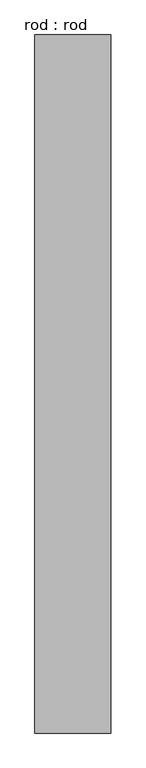
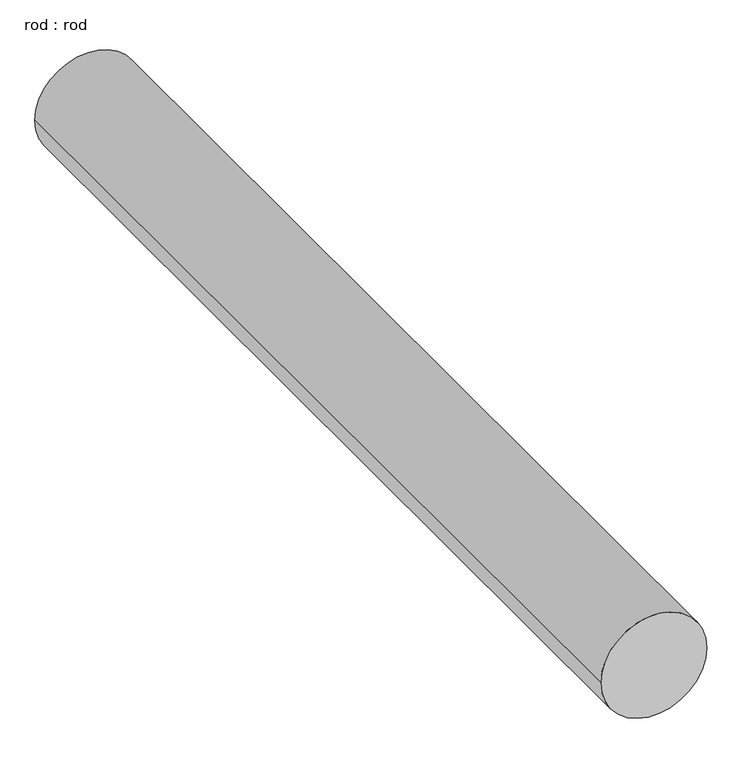
"""IFC4 building model written with IfcOpenShell, lengths in millimetres: proxy geometry, rod : rod."""

from ifc_helpers import new_model, si_unit, point, frame, frame_2d, origin, place, context, project, spatial, circle_curve, trimmed, segment, composite_curve, outline, extrude, source, transform, mapped, element, save


def rod_rod_663d910f(model_context):
    return source(origin(), model_context, "Body", "SweptSolid", [
        extrude(outline(composite_curve([segment(trimmed(circle_curve(frame_2d((0.0108462, 0.0)), 200.0), [point((0.0108462, 200.0))], [point((0.0108462, -200.0))], False, "CARTESIAN"), True, "CONTINUOUS"), segment(trimmed(circle_curve(frame_2d((0.0108462, 0.0)), 200.0), [point((0.0108462, -200.0))], [point((0.0108462, 200.0))], False, "CARTESIAN"), True, "CONTINUOUS")], self_intersect=False)), frame((0.0, 2247.8556522, 0.0), z_axis=(0.0, 1.0, 0.0), x_axis=(0.0, 0.0, 1.0)), (0.0, 0.0, 1.0), 3689.7459262),
    ])


if __name__ == "__main__":
    model = new_model("IFC4")
    model_context = context("Model", 3, world=origin())
    ifc_project = project(units=[si_unit("LENGTHUNIT", "METRE", prefix="MILLI")], contexts=[model_context])
    site = spatial("IfcSite", under=ifc_project)
    building = spatial("IfcBuilding", under=site)
    placement = place(None, origin())
    rod_rod_shape = rod_rod_663d910f(model_context)
    element("IfcBuildingElementProxy", 1, Name="rod : rod", ObjectType="rod : rod", at=placement, inside=building, context=model_context, shape_type="MappedRepresentation", body=[
        mapped(rod_rod_shape, transform((0.0, 0.0, 0.0), x_axis=(1.0, 0.0, 0.0), y_axis=(0.0, 1.0, 0.0), z_axis=(0.0, 0.0, 1.0))),
    ])
    save(model, "model.ifc")

# Revit data of these elements
# Type "rod : rod"
#   Default Elevation = 0
